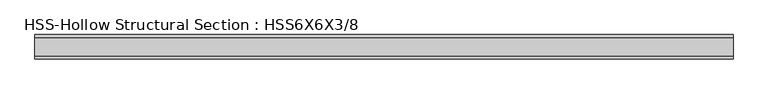
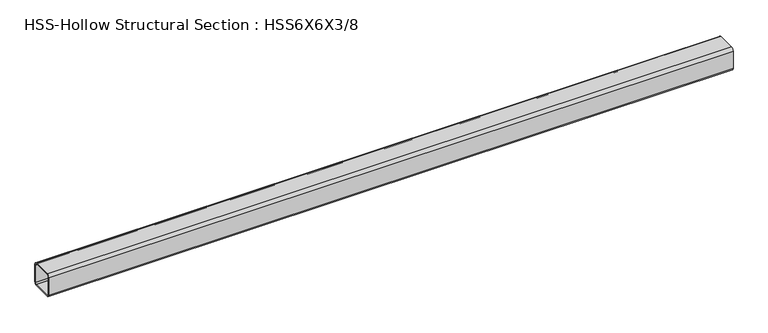
"""IFC4 building model written with IfcOpenShell, lengths in millimetres: member geometry, HSS-Hollow Structural Section : HSS6X6X3/8."""

from ifc_helpers import new_model, si_unit, point, frame, frame_2d, origin, place, context, project, spatial, polyline, circle_curve, trimmed, segment, composite_curve, outline, extrude, source, transform, mapped, element, save


def hss_hollow_structural_section_hss6x6x3_8_4800b8b9(model_context):
    return source(origin(), model_context, "Body", "SweptSolid", [
        extrude(outline(composite_curve([segment(polyline([(76.2, 58.4708), (76.2, -58.4708)]), True, "CONTINUOUS"), segment(trimmed(circle_curve(frame_2d((58.4708, -58.4708)), 17.7292), [point((76.2, -58.4708))], [point((58.4708, -76.2))], False, "CARTESIAN"), True, "CONTINUOUS"), segment(polyline([(58.4708, -76.2), (-58.4708, -76.2)]), True, "CONTINUOUS"), segment(trimmed(circle_curve(frame_2d((-58.4708, -58.4708)), 17.7292), [point((-58.4708, -76.2))], [point((-76.2, -58.4708))], False, "CARTESIAN"), True, "CONTINUOUS"), segment(polyline([(-76.2, -58.4708), (-76.2, 58.4708)]), True, "CONTINUOUS"), segment(trimmed(circle_curve(frame_2d((-58.4708, 58.4708)), 17.7292), [point((-76.2, 58.4708))], [point((-58.4708, 76.2))], False, "CARTESIAN"), True, "CONTINUOUS"), segment(polyline([(-58.4708, 76.2), (58.4708, 76.2)]), True, "CONTINUOUS"), segment(trimmed(circle_curve(frame_2d((58.4708, 58.4708)), 17.7292), [point((58.4708, 76.2))], [point((76.2, 58.4708))], False, "CARTESIAN"), True, "CONTINUOUS")], self_intersect=False), holes=[composite_curve([segment(trimmed(circle_curve(frame_2d((-58.4708, 58.4708)), 8.8646), [point((-58.4708, 67.3354))], [point((-67.3354, 58.4708))], True, "CARTESIAN"), True, "CONTINUOUS"), segment(polyline([(-67.3354, 58.4708), (-67.3354, -58.4708)]), True, "CONTINUOUS"), segment(trimmed(circle_curve(frame_2d((-58.4708, -58.4708)), 8.8646), [point((-67.3354, -58.4708))], [point((-58.4708, -67.3354))], True, "CARTESIAN"), True, "CONTINUOUS"), segment(polyline([(-58.4708, -67.3354), (58.4708, -67.3354)]), True, "CONTINUOUS"), segment(trimmed(circle_curve(frame_2d((58.4708, -58.4708)), 8.8646), [point((58.4708, -67.3354))], [point((67.3354, -58.4708))], True, "CARTESIAN"), True, "CONTINUOUS"), segment(polyline([(67.3354, -58.4708), (67.3354, 58.4708)]), True, "CONTINUOUS"), segment(trimmed(circle_curve(frame_2d((58.4708, 58.4708)), 8.8646), [point((67.3354, 58.4708))], [point((58.4708, 67.3354))], True, "CARTESIAN"), True, "CONTINUOUS"), segment(polyline([(58.4708, 67.3354), (-58.4708, 67.3354)]), True, "CONTINUOUS")], self_intersect=False)]), frame((-2206.6695731, 0.0, 0.0), z_axis=(1.0, 0.0, 0.0), x_axis=(0.0, 1.0, 0.0)), (0.0, 0.0, 1.0), 4393.6395374),
    ])


if __name__ == "__main__":
    model = new_model("IFC4")
    model_context = context("Model", 3, world=origin())
    ifc_project = project(units=[si_unit("LENGTHUNIT", "METRE", prefix="MILLI")], contexts=[model_context])
    site = spatial("IfcSite", under=ifc_project)
    building = spatial("IfcBuilding", under=site)
    placement = place(None, origin())
    hss_hollow_structural_section_hss6x6x3_8_shape = hss_hollow_structural_section_hss6x6x3_8_4800b8b9(model_context)
    element("IfcMember", 1, ObjectType="HSS-Hollow Structural Section : HSS6X6X3/8", at=placement, inside=building, context=model_context, shape_type="MappedRepresentation", body=[
        mapped(hss_hollow_structural_section_hss6x6x3_8_shape, transform((0.0, 0.0, 0.0), x_axis=(1.0, 0.0, 0.0), y_axis=(0.0, 1.0, 0.0), z_axis=(0.0, 0.0, 1.0))),
    ])
    save(model, "model.ifc")

# Revit data of these elements
# Type "HSS-Hollow Structural Section : HSS6X6X3/8"
#   Assembly Code = "B10"
#   Shape = "Square"
#   W = 27.4
#   Ht = 0' - 6"
#   Length [instance default] = 5' - 0"
#   b = 0' - 6"
#   kr = 0' - 0.698"
#   t = 0' - 0.349"
#   A = 0.0526389 SF
#   Structural Material [instance default] = Steel ASTM A500, Grade B, Rectangular and Square
# Element 1 (IfcMember, "HSS-Hollow Structural Section : HSS6X6X3/8")
#   Materials on its faces: "Steel ASTM A500, Grade B, Rectangular and Square"
# Materials
#   "Steel ASTM A500, Grade B, Rectangular and Square": class "Metal", colour RGB 199 199 199, transparency 0, Description = "Carbon steel", Cost = 0
